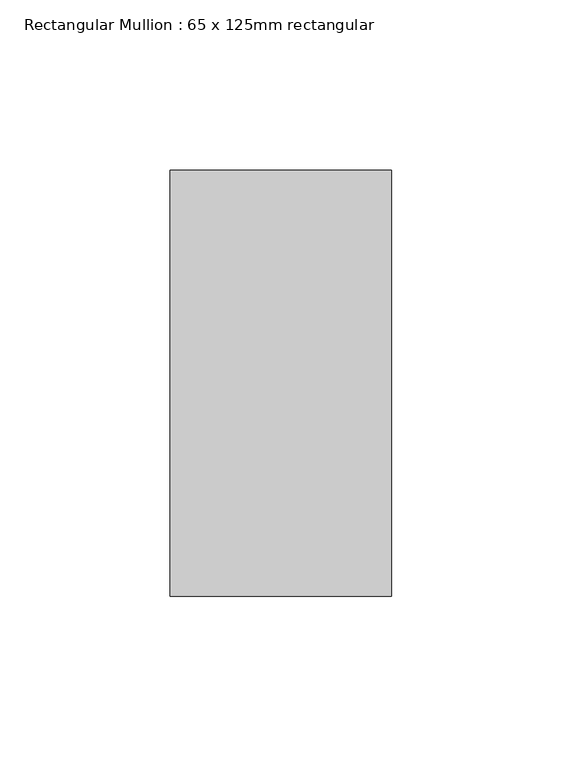
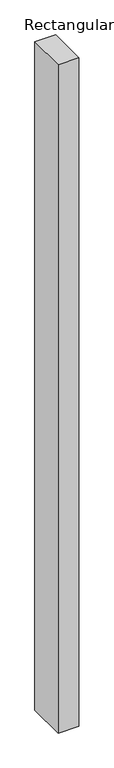
"""IFC4 building model written with IfcOpenShell, lengths in millimetres: member geometry, Rectangular Mullion : 65 x 125mm rectangular."""

from ifc_helpers import new_model, si_unit, frame, origin, place, context, project, spatial, polyline, outline, extrude, source, transform, mapped, element, save


def rectangular_mullion_65_x_125mm_rectangular_02dc2359(model_context):
    return source(origin(), model_context, "Body", "SweptSolid", [
        extrude(outline(polyline([(0.0, 62.5), (0.0, -62.5), (-65.0, -62.5), (-65.0, 62.5), (0.0, 62.5)])), frame((0.0, 0.0, -2200.0), z_axis=(0.0, 0.0, 1.0), x_axis=(1.0, 0.0, 0.0)), (0.0, 0.0, 1.0), 2200.0),
    ])


if __name__ == "__main__":
    model = new_model("IFC4")
    model_context = context("Model", 3, world=origin())
    ifc_project = project(units=[si_unit("LENGTHUNIT", "METRE", prefix="MILLI")], contexts=[model_context])
    site = spatial("IfcSite", under=ifc_project)
    building = spatial("IfcBuilding", under=site)
    placement = place(None, origin())
    rectangular_mullion_65_x_125mm_rectangular_shape = rectangular_mullion_65_x_125mm_rectangular_02dc2359(model_context)
    element("IfcMember", 1, ObjectType="Rectangular Mullion : 65 x 125mm rectangular", at=placement, inside=building, context=model_context, shape_type="MappedRepresentation", body=[
        mapped(rectangular_mullion_65_x_125mm_rectangular_shape, transform((0.0, 0.0, 0.0), x_axis=(1.0, 0.0, 0.0), y_axis=(0.0, 1.0, 0.0), z_axis=(0.0, 0.0, 1.0))),
    ])
    save(model, "model.ifc")

# Revit data of these elements
# Type "Rectangular Mullion : 65 x 125mm rectangular"
#   built-in parameter 1007304 = 0.410105 (stored number, unit not read)
#   built-in parameter 1007301 = 0.106627 (stored number, unit not read)
#   built-in parameter 1007300 = 0.106627 (stored number, unit not read)
# Element 1 (IfcMember, "Rectangular Mullion : 65 x 125mm rectangular")
#   Materials on its faces: "Aluminum"
# Materials
#   "Aluminum": class "Metal", colour RGB 244 245 246, transparency 0, Description = "Aluminum 6061", Cost = 0
